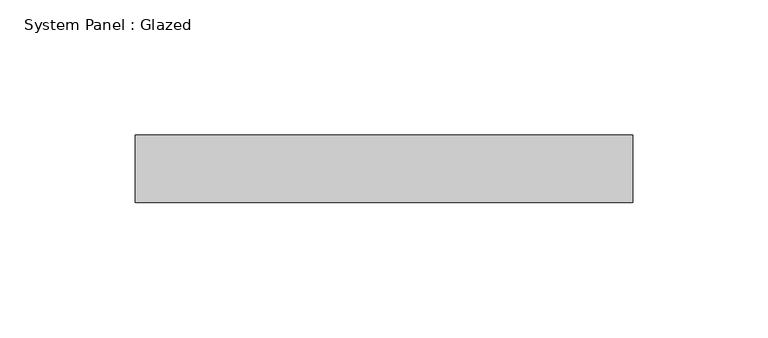
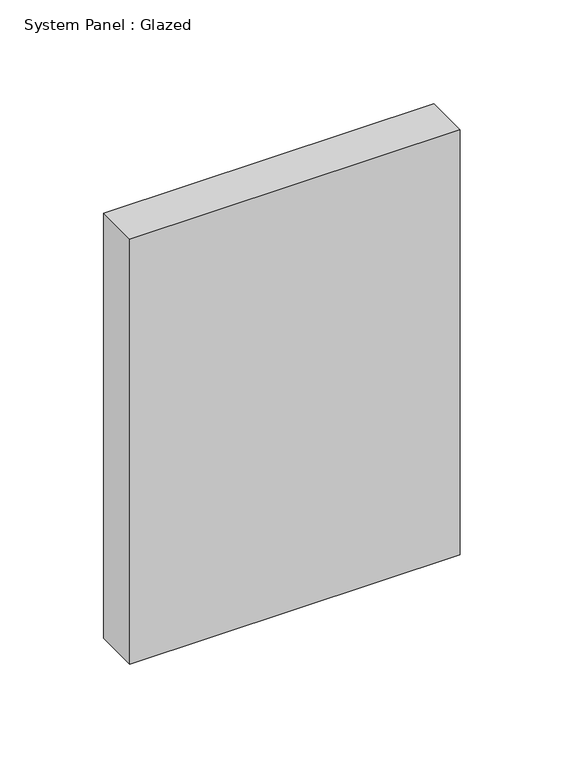
"""IFC4 building model written with IfcOpenShell, lengths in millimetres: plate geometry, System Panel : Glazed."""

from ifc_helpers import new_model, si_unit, origin, origin_with_axes, place, context, project, spatial, polyline, outline, extrude, source, transform, mapped, element, save


def system_panel_glazed_e80698b1(model_context):
    return source(origin(), model_context, "Body", "SweptSolid", [
        extrude(outline(polyline([(91.9191919, 24.5), (-91.9191919, 24.5), (-91.9191919, 49.5), (91.9191919, 49.5), (91.9191919, 24.5)])), origin_with_axes(), (0.0, 0.0, 1.0), 250.0),
    ])


if __name__ == "__main__":
    model = new_model("IFC4")
    model_context = context("Model", 3, world=origin())
    ifc_project = project(units=[si_unit("LENGTHUNIT", "METRE", prefix="MILLI")], contexts=[model_context])
    site = spatial("IfcSite", under=ifc_project)
    building = spatial("IfcBuilding", under=site)
    placement = place(None, origin())
    system_panel_glazed_shape = system_panel_glazed_e80698b1(model_context)
    element("IfcPlate", 1, ObjectType="System Panel : Glazed", at=placement, inside=building, context=model_context, shape_type="MappedRepresentation", body=[
        mapped(system_panel_glazed_shape, transform((0.0, 0.0, 0.0), x_axis=(1.0, 0.0, 0.0), y_axis=(0.0, 1.0, 0.0), z_axis=(0.0, 0.0, 1.0))),
    ])
    save(model, "model.ifc")

# Revit data of these elements
# Element 1 (IfcPlate, "System Panel : Glazed")
#   Materials on its faces: "Glass"
# Materials
#   "Glass": class "Glass", colour RGB 218 227 224, transparency 0.85, Description = "Soda Lime Glass", Cost = 0
